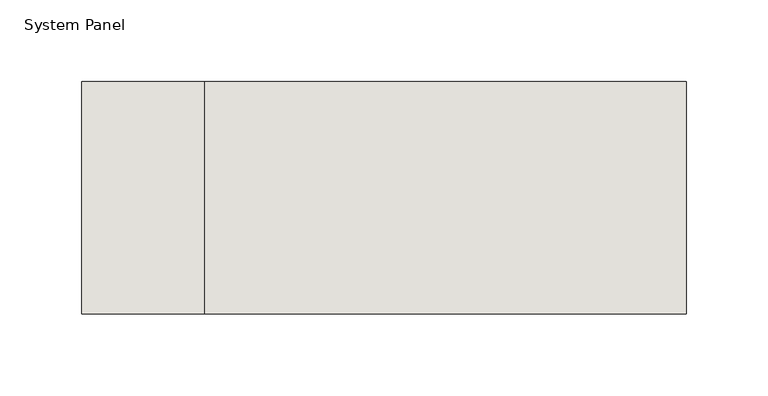
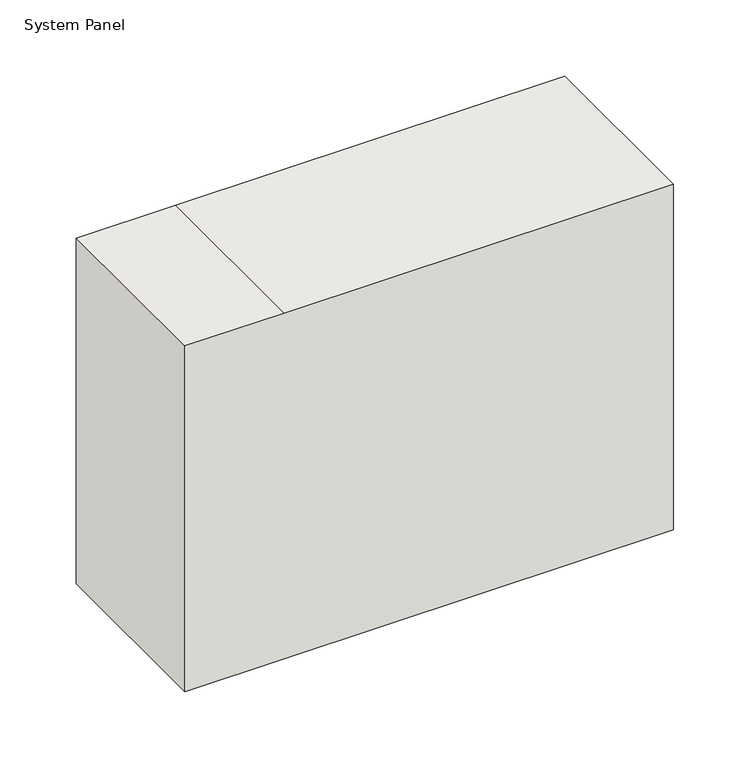
"""IFC4 building model written with IfcOpenShell, lengths in millimetres: wall geometry, System Panel : NLRS_21_CWP_hsb-vulling minerale wol 142 _gen_rsf."""

from ifc_helpers import new_model, si_unit, frame, origin, place, context, project, spatial, polyline, outline, extrude, source, transform, mapped, element, save


def system_panel_37dbae85(model_context):
    return source(origin(), model_context, "Body", "SweptSolid", [
        extrude(outline(polyline([(0.0, -184.5), (0.0, -109.3441061), (0.0, 184.5), (276.0, 184.5), (276.0, -109.3441061), (276.0, -184.5), (0.0, -184.5)])), frame((0.0, -71.0, 0.0), z_axis=(0.0, 1.0, 0.0), x_axis=(0.0, 0.0, 1.0)), (0.0, 0.0, 1.0), 142.0),
    ])


if __name__ == "__main__":
    model = new_model("IFC4")
    model_context = context("Model", 3, world=origin())
    ifc_project = project(units=[si_unit("LENGTHUNIT", "METRE", prefix="MILLI")], contexts=[model_context])
    site = spatial("IfcSite", under=ifc_project)
    building = spatial("IfcBuilding", under=site)
    placement = place(None, origin())
    system_panel_shape = system_panel_37dbae85(model_context)
    element("IfcWall", 1, ObjectType="System Panel : NLRS_21_CWP_hsb-vulling minerale wol 142 _gen_rsf", at=placement, inside=building, context=model_context, shape_type="MappedRepresentation", body=[
        mapped(system_panel_shape, transform((0.0, 0.0, 0.0), x_axis=(1.0, 0.0, 0.0), y_axis=(0.0, 1.0, 0.0), z_axis=(0.0, 0.0, 1.0))),
    ])
    save(model, "model.ifc")

# Revit data of these elements
# Type "System Panel : NLRS_21_CWP_hsb-vulling minerale wol 142 _gen_rsf"
#   Type IfcGUID = "07M7mRoiH1CR8m_RSKIwpC"
#   Assembly Code = "21.23"
#   IfcExportAs = "IfcWall"
# Element 1 (IfcWall, "System Panel : NLRS_21_CWP_hsb-vulling minerale wol 142 _gen_rsf")
#   Materials on its faces: "NLRS_m1_isolatie minerale wol_gen_rsf"
# Materials
#   "NLRS_m1_isolatie minerale wol_gen_rsf": class "M - Anorganische materialen", colour RGB 200 200 140, transparency 0, Keynote = "m1", Manufacturer = "Revit Standards Foundation", URL = "www.revitstandards.org", Description = "isolatie minerale wol", Cost = 0
